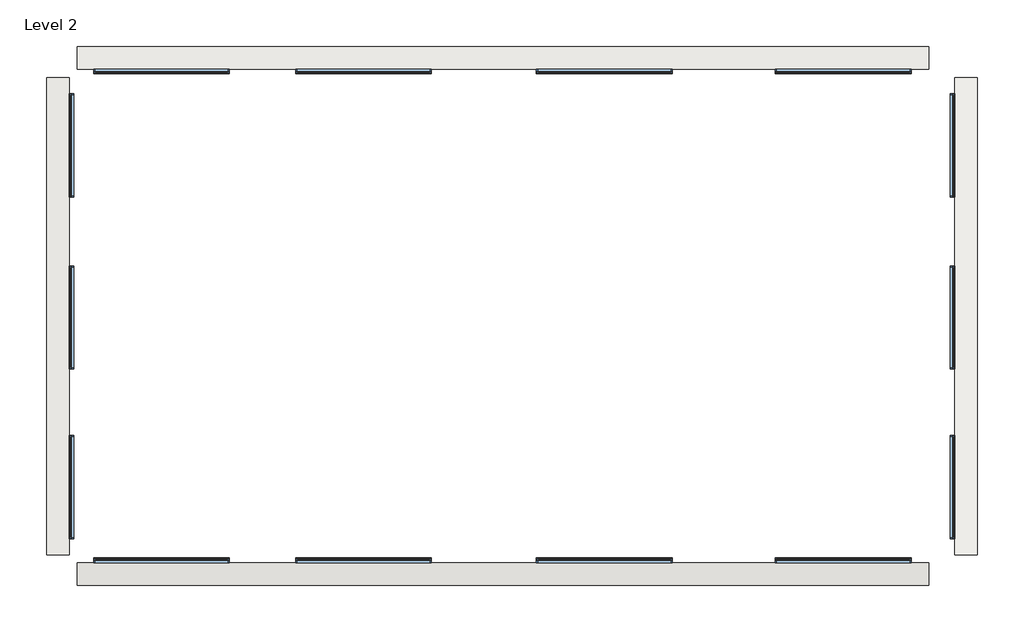
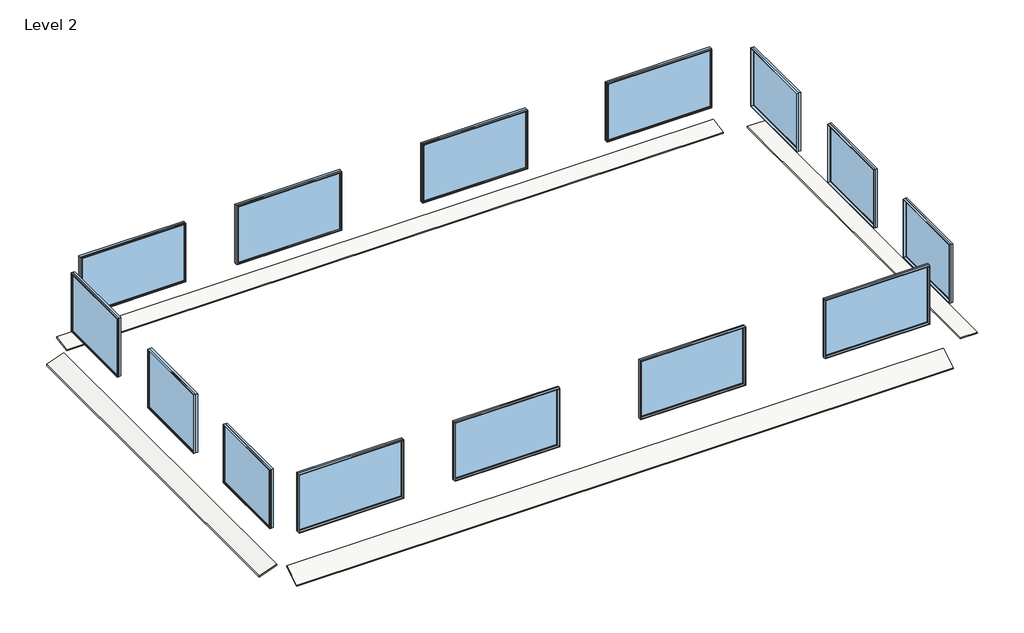
# One storey: 14 windows, 4 roofs.
"""IFC4 building model written with IfcOpenShell, lengths in millimetres."""

import ifcopenshell
import ifcopenshell.guid

model = None  # the IFC model being written
_history = None  # IfcOwnerHistory: only IFC2X3 demands one
_inside = {}  # id of a spatial element -> (the spatial element, [elements in it])
_under = {}  # id of a project, library or spatial element -> (it, [spatial elements below it])
_declared = {}  # id of a project -> (the project, [libraries it declares])
_typed = {}  # id of a type object -> (the type object, [elements of that type])
_made_of = {}  # id of a material, layer set ... -> (it, [elements and type objects made of it])


def new_model(schema):
    """Start an empty IFC model of exactly this schema.

    Asked for "IFC4X3", IfcOpenShell would pick the latest addendum, in which some entities
    have other attributes; the version numbers below select the first issue.
    IFC2X3 requires an IfcOwnerHistory on every rooted entity: one is made here for all.
    """
    global model, _history
    if schema == "IFC4X3":
        model = ifcopenshell.file(schema_version=(4, 3, 0, 0))
    else:
        model = ifcopenshell.file(schema=schema)
    _inside.clear()
    _under.clear()
    _declared.clear()
    _typed.clear()
    _made_of.clear()
    _history = None
    if model.schema == "IFC2X3":
        org = make("IfcOrganization", Name="unknown")
        user = make(
            "IfcPersonAndOrganization",
            ThePerson=make("IfcPerson", FamilyName="unknown"),
            TheOrganization=org,
        )
        app = make(
            "IfcApplication",
            ApplicationDeveloper=org,
            Version="unknown",
            ApplicationFullName="unknown",
            ApplicationIdentifier="unknown",
        )
        _history = make(
            "IfcOwnerHistory",
            OwningUser=user,
            OwningApplication=app,
            ChangeAction="ADDED",
            CreationDate=0,
        )
    return model


def make(cls, **values):
    """One entity of the class cls with the attributes given. An attribute that is None is left unset."""
    return model.create_entity(
        cls, **{name: value for name, value in values.items() if value is not None}
    )


def rooted(cls, **values):
    """An entity with a GlobalId (a new one), such as an element, a storey or a relation."""
    return make(cls, GlobalId=ifcopenshell.guid.new(), OwnerHistory=_history, **values)


def si_unit(unit_type, name, prefix=None):
    """IfcSIUnit, for example si_unit("LENGTHUNIT", "METRE", prefix="MILLI")."""
    return make("IfcSIUnit", UnitType=unit_type, Prefix=prefix, Name=name)


def assignment(units):
    """IfcUnitAssignment: the units of a project."""
    return None if units is None else make("IfcUnitAssignment", Units=units)


def point(xyz):
    """IfcCartesianPoint."""
    return None if xyz is None else make("IfcCartesianPoint", Coordinates=xyz)


def direction(xyz):
    """IfcDirection."""
    return None if xyz is None else make("IfcDirection", DirectionRatios=xyz)


def frame(location, z_axis=None, x_axis=None):
    """IfcAxis2Placement3D, a coordinate frame: its origin and axes. An axis left out is left unset."""
    return make(
        "IfcAxis2Placement3D",
        Location=point(location),
        Axis=direction(z_axis),
        RefDirection=direction(x_axis),
    )


def origin():
    """The frame at (0, 0, 0) with its axes left unset."""
    return frame((0.0, 0.0, 0.0))


def place(relative_to, where):
    """IfcLocalPlacement: puts the frame where relative to a parent placement (None: the world)."""
    return make(
        "IfcLocalPlacement", PlacementRelTo=relative_to, RelativePlacement=where
    )


def context(
    kind, dimensions, precision=None, world=None, true_north=None, identifier=None
):
    """IfcGeometricRepresentationContext, for example the 3D "Model" context."""
    return make(
        "IfcGeometricRepresentationContext",
        ContextIdentifier=identifier,
        ContextType=kind,
        CoordinateSpaceDimension=dimensions,
        Precision=precision,
        WorldCoordinateSystem=world,
        TrueNorth=true_north,
    )


def project(units=None, contexts=None):
    """IfcProject with its units and contexts."""
    return rooted(
        "IfcProject",
        Name="project",
        RepresentationContexts=contexts,
        UnitsInContext=assignment(units),
    )


def spatial(cls, under=None, at=None, **own):
    """A site, building, storey or space (cls), placed at a placement, below another one or the project."""
    s = rooted(cls, ObjectPlacement=at, **own)
    if under is not None:
        _under.setdefault(under.id(), (under, []))[1].append(s)
    return s


def polyline(points):
    """IfcPolyline through the points."""
    return make("IfcPolyline", Points=[point(p) for p in points])


def outline(outer, holes=None, kind="AREA"):
    """IfcArbitraryClosedProfileDef: a profile drawn as a closed curve; with holes, ...WithVoids."""
    if holes is None:
        return make("IfcArbitraryClosedProfileDef", ProfileType=kind, OuterCurve=outer)
    return make(
        "IfcArbitraryProfileDefWithVoids",
        ProfileType=kind,
        OuterCurve=outer,
        InnerCurves=holes,
    )


def extrude(swept, where, along, depth):
    """IfcExtrudedAreaSolid: the profile swept, set in the frame where, extruded along a direction by depth."""
    return make(
        "IfcExtrudedAreaSolid",
        SweptArea=swept,
        Position=where,
        ExtrudedDirection=direction(along),
        Depth=depth,
    )


def shape(context_of_items, identifier, shape_type, items):
    """IfcShapeRepresentation: the items that make up one representation, for example the "Body"."""
    return make(
        "IfcShapeRepresentation",
        ContextOfItems=context_of_items,
        RepresentationIdentifier=identifier,
        RepresentationType=shape_type,
        Items=items,
    )


def source(mapping_origin, context_of_items, identifier, shape_type, items):
    """IfcRepresentationMap: a shape defined once, which mapped items show again and again."""
    return make(
        "IfcRepresentationMap",
        MappingOrigin=mapping_origin,
        MappedRepresentation=shape(context_of_items, identifier, shape_type, items),
    )


def transform(
    local_origin,
    x_axis=None,
    y_axis=None,
    z_axis=None,
    scale=None,
    scale2=None,
    scale3=None,
    uniform=True,
):
    """IfcCartesianTransformationOperator3D, or its non-uniform kind. x_axis, y_axis, z_axis: its Axis1, 2, 3."""
    if uniform:
        return make(
            "IfcCartesianTransformationOperator3D",
            Axis1=direction(x_axis),
            Axis2=direction(y_axis),
            LocalOrigin=point(local_origin),
            Scale=scale,
            Axis3=direction(z_axis),
        )
    return make(
        "IfcCartesianTransformationOperator3DnonUniform",
        Axis1=direction(x_axis),
        Axis2=direction(y_axis),
        LocalOrigin=point(local_origin),
        Scale=scale,
        Axis3=direction(z_axis),
        Scale2=scale2,
        Scale3=scale3,
    )


def mapped(mapping_source, mapping_target):
    """IfcMappedItem: shows the shape of a source again, moved by a transform."""
    return make(
        "IfcMappedItem", MappingSource=mapping_source, MappingTarget=mapping_target
    )


def made_of(thing, what):
    """Note that an element or type object is made of a material, layer set ...; save() writes the relation."""
    if what is not None:
        _made_of.setdefault(what.id(), (what, []))[1].append(thing)
    return thing


def element(
    cls,
    number,
    at=None,
    inside=None,
    cuts=None,
    type_object=None,
    material=None,
    context=None,
    identifier="Body",
    shape_type=None,
    held_by="IfcProductDefinitionShape",
    body=None,
    shapes=None,
    **own,
):
    """One element of the class cls, such as IfcWall. Its Tag is "e" and its number.

    at: its placement. inside: the storey or other place that contains it. cuts: it is an
    opening in that element (IfcRelVoidsElement). A single representation is given by context,
    identifier, shape_type and body (its items); several are given by shapes. held_by: the class
    of the entity that holds the representations. save() writes the other relations.
    """
    e = rooted(cls, Tag="e%d" % number, ObjectPlacement=at, **own)
    if body is not None:
        shapes = [shape(context, identifier, shape_type, body)]
    if shapes is not None:
        e.Representation = make(held_by, Representations=shapes)
    if inside is not None:
        _inside.setdefault(inside.id(), (inside, []))[1].append(e)
    if cuts is not None:
        rooted(
            "IfcRelVoidsElement", RelatingBuildingElement=cuts, RelatedOpeningElement=e
        )
    if type_object is not None:
        _typed.setdefault(type_object.id(), (type_object, []))[1].append(e)
    return made_of(e, material)


def aggregate(whole, parts):
    """IfcRelAggregates: a whole, such as a stair, and the parts it consists of."""
    return rooted("IfcRelAggregates", RelatingObject=whole, RelatedObjects=parts)


def save(model, path):
    """Write the relations noted so far, then the file.

    IfcRelAggregates (storeys below a building ...), IfcRelContainedInSpatialStructure (elements
    in a storey), IfcRelDefinesByType, IfcRelAssociatesMaterial and IfcRelDeclares: one each for
    every whole, place, type object, material and project.
    """
    for whole, parts in _under.values():
        aggregate(whole, parts)
    for where, things in _inside.values():
        rooted(
            "IfcRelContainedInSpatialStructure",
            RelatedElements=things,
            RelatingStructure=where,
        )
    for kind, things in _typed.values():
        rooted("IfcRelDefinesByType", RelatedObjects=things, RelatingType=kind)
    for what, things in _made_of.values():
        rooted("IfcRelAssociatesMaterial", RelatedObjects=things, RelatingMaterial=what)
    for by, libraries in _declared.values():
        rooted("IfcRelDeclares", RelatingContext=by, RelatedDefinitions=libraries)
    model.write(path)


def m_fixed_2500x_4228mm_fd5e51e7(model_context):
    return source(origin(), model_context, "Body", "SweptSolid", [
        extrude(outline(polyline([(-2050.8, 54.2), (2050.8, 54.2), (2050.8, 42.2), (-2050.8, 42.2), (-2050.8, 54.2)])), frame((0.0, 0.0, 368.0), z_axis=(0.0, 0.0, 1.0), x_axis=(1.0, 0.0, 0.0)), (0.0, 0.0, 1.0), 2374.0),
        extrude(outline(polyline([(2786.0, -2094.8), (324.0, -2094.8), (324.0, 2094.8), (2786.0, 2094.8), (2786.0, -2094.8)]), holes=[polyline([(2742.0, -2050.8), (2742.0, 2050.8), (368.0, 2050.8), (368.0, -2050.8), (2742.0, -2050.8)])]), frame((0.0, 26.2, 0.0), z_axis=(0.0, 1.0, 0.0), x_axis=(0.0, 0.0, 1.0)), (0.0, 0.0, 1.0), 44.0),
        extrude(outline(polyline([(2805.0, -2113.8), (305.0, -2113.8), (305.0, 2113.8), (2805.0, 2113.8), (2805.0, -2113.8)]), holes=[polyline([(2786.0, -2094.8), (2786.0, 2094.8), (324.0, 2094.8), (324.0, -2094.8), (2786.0, -2094.8)])]), frame((0.0, 26.2, 0.0), z_axis=(0.0, 1.0, 0.0), x_axis=(0.0, 0.0, 1.0)), (0.0, 0.0, 1.0), 63.0),
        extrude(outline(polyline([(2805.0, -2113.8), (305.0, -2113.8), (305.0, 2113.8), (2805.0, 2113.8), (2805.0, -2113.8)]), holes=[polyline([(2773.0, -2081.8), (2773.0, 2081.8), (337.0, 2081.8), (337.0, -2081.8), (2773.0, -2081.8)])]), frame((0.0, -63.2, 0.0), z_axis=(0.0, 1.0, 0.0), x_axis=(0.0, 0.0, 1.0)), (0.0, 0.0, 1.0), 89.4),
    ])


def m_fixed_2500x_4228mm_f14c179f(model_context):
    return source(origin(), model_context, "Body", "SweptSolid", [
        extrude(outline(polyline([(-2050.8, -54.2), (-2050.8, -42.2), (2050.8, -42.2), (2050.8, -54.2), (-2050.8, -54.2)])), frame((0.0, 0.0, 368.0), z_axis=(0.0, 0.0, 1.0), x_axis=(1.0, 0.0, 0.0)), (0.0, 0.0, 1.0), 2374.0),
        extrude(outline(polyline([(2786.0, -2094.8), (324.0, -2094.8), (324.0, 2094.8), (2786.0, 2094.8), (2786.0, -2094.8)]), holes=[polyline([(2742.0, -2050.8), (2742.0, 2050.8), (368.0, 2050.8), (368.0, -2050.8), (2742.0, -2050.8)])]), frame((0.0, -70.2, 0.0), z_axis=(0.0, 1.0, 0.0), x_axis=(0.0, 0.0, 1.0)), (0.0, 0.0, 1.0), 44.0),
        extrude(outline(polyline([(2805.0, -2113.8), (305.0, -2113.8), (305.0, 2113.8), (2805.0, 2113.8), (2805.0, -2113.8)]), holes=[polyline([(2786.0, -2094.8), (2786.0, 2094.8), (324.0, 2094.8), (324.0, -2094.8), (2786.0, -2094.8)])]), frame((0.0, -89.2, 0.0), z_axis=(0.0, 1.0, 0.0), x_axis=(0.0, 0.0, 1.0)), (0.0, 0.0, 1.0), 63.0),
        extrude(outline(polyline([(2805.0, -2113.8), (305.0, -2113.8), (305.0, 2113.8), (2805.0, 2113.8), (2805.0, -2113.8)]), holes=[polyline([(2773.0, -2081.8), (2773.0, 2081.8), (337.0, 2081.8), (337.0, -2081.8), (2773.0, -2081.8)])]), frame((0.0, -26.2, 0.0), z_axis=(0.0, 1.0, 0.0), x_axis=(0.0, 0.0, 1.0)), (0.0, 0.0, 1.0), 89.4),
    ])


def m_fixed_2500x_3220mm_df94f4d0(model_context):
    return source(origin(), model_context, "Body", "SweptSolid", [
        extrude(outline(polyline([(-1546.8, 54.2), (1546.8, 54.2), (1546.8, 42.2), (-1546.8, 42.2), (-1546.8, 54.2)])), frame((0.0, 0.0, 368.0), z_axis=(0.0, 0.0, 1.0), x_axis=(1.0, 0.0, 0.0)), (0.0, 0.0, 1.0), 2374.0),
        extrude(outline(polyline([(2786.0, -1590.8), (324.0, -1590.8), (324.0, 1590.8), (2786.0, 1590.8), (2786.0, -1590.8)]), holes=[polyline([(2742.0, -1546.8), (2742.0, 1546.8), (368.0, 1546.8), (368.0, -1546.8), (2742.0, -1546.8)])]), frame((0.0, 26.2, 0.0), z_axis=(0.0, 1.0, 0.0), x_axis=(0.0, 0.0, 1.0)), (0.0, 0.0, 1.0), 44.0),
        extrude(outline(polyline([(2805.0, -1609.8), (305.0, -1609.8), (305.0, 1609.8), (2805.0, 1609.8), (2805.0, -1609.8)]), holes=[polyline([(2786.0, -1590.8), (2786.0, 1590.8), (324.0, 1590.8), (324.0, -1590.8), (2786.0, -1590.8)])]), frame((0.0, 26.2, 0.0), z_axis=(0.0, 1.0, 0.0), x_axis=(0.0, 0.0, 1.0)), (0.0, 0.0, 1.0), 63.0),
        extrude(outline(polyline([(2805.0, -1609.8), (305.0, -1609.8), (305.0, 1609.8), (2805.0, 1609.8), (2805.0, -1609.8)]), holes=[polyline([(2773.0, -1577.8), (2773.0, 1577.8), (337.0, 1577.8), (337.0, -1577.8), (2773.0, -1577.8)])]), frame((0.0, -63.2, 0.0), z_axis=(0.0, 1.0, 0.0), x_axis=(0.0, 0.0, 1.0)), (0.0, 0.0, 1.0), 89.4),
    ])


def m_fixed_2500x_3220mm_8b997f8c(model_context):
    return source(origin(), model_context, "Body", "SweptSolid", [
        extrude(outline(polyline([(-1546.8, -54.2), (-1546.8, -42.2), (1546.8, -42.2), (1546.8, -54.2), (-1546.8, -54.2)])), frame((0.0, 0.0, 368.0), z_axis=(0.0, 0.0, 1.0), x_axis=(1.0, 0.0, 0.0)), (0.0, 0.0, 1.0), 2374.0),
        extrude(outline(polyline([(2786.0, -1590.8), (324.0, -1590.8), (324.0, 1590.8), (2786.0, 1590.8), (2786.0, -1590.8)]), holes=[polyline([(2742.0, -1546.8), (2742.0, 1546.8), (368.0, 1546.8), (368.0, -1546.8), (2742.0, -1546.8)])]), frame((0.0, -70.2, 0.0), z_axis=(0.0, 1.0, 0.0), x_axis=(0.0, 0.0, 1.0)), (0.0, 0.0, 1.0), 44.0),
        extrude(outline(polyline([(2805.0, -1609.8), (305.0, -1609.8), (305.0, 1609.8), (2805.0, 1609.8), (2805.0, -1609.8)]), holes=[polyline([(2786.0, -1590.8), (2786.0, 1590.8), (324.0, 1590.8), (324.0, -1590.8), (2786.0, -1590.8)])]), frame((0.0, -89.2, 0.0), z_axis=(0.0, 1.0, 0.0), x_axis=(0.0, 0.0, 1.0)), (0.0, 0.0, 1.0), 63.0),
        extrude(outline(polyline([(2805.0, -1609.8), (305.0, -1609.8), (305.0, 1609.8), (2805.0, 1609.8), (2805.0, -1609.8)]), holes=[polyline([(2773.0, -1577.8), (2773.0, 1577.8), (337.0, 1577.8), (337.0, -1577.8), (2773.0, -1577.8)])]), frame((0.0, -26.2, 0.0), z_axis=(0.0, 1.0, 0.0), x_axis=(0.0, 0.0, 1.0)), (0.0, 0.0, 1.0), 89.4),
    ])


model = new_model("IFC4")

# Units and contexts
model_context = context("Model", 3, world=origin())
ifc_project = project(units=[si_unit("LENGTHUNIT", "METRE", prefix="MILLI")], contexts=[model_context])

# Site, building, storey
site = spatial("IfcSite", under=ifc_project)
building = spatial("IfcBuilding", under=site)
storey = spatial("IfcBuildingStorey", under=building, Name="Level 2", Elevation=3962.4)

# Roofs
placement = place(None, origin())
element("IfcRoof", 1, ObjectType="Shading devices - 50mm", at=placement, inside=storey, context=model_context, shape_type="SweptSolid", body=[
    extrude(outline(polyline([(-4795.4197783, 3248.2548116), (-4095.4197783, 3652.4), (-4095.4197783, 3594.6649731), (-4795.4197783, 3190.5197846), (-4795.4197783, 3248.2548116)])), frame((1746.464681, 0.0, 0.0), z_axis=(1.0, 0.0, 0.0), x_axis=(0.0, 1.0, 0.0)), (0.0, 0.0, 1.0), 26500.0),
])
element("IfcRoof", 2, ObjectType="Shading devices - 50mm", at=placement, inside=storey, context=model_context, shape_type="SweptSolid", body=[
    extrude(outline(polyline([(29068.464681, 11030.5802217), (29768.464681, 11030.5802217), (29768.464681, -3843.0197783), (29068.464681, -3843.0197783), (29068.464681, 11030.5802217)])), frame((0.0, 0.0, 3602.4), z_axis=(0.0, 0.0, 1.0), x_axis=(1.0, 0.0, 0.0)), (0.0, 0.0, 1.0), 50.0),
])
element("IfcRoof", 3, ObjectType="Shading devices - 50mm", at=placement, inside=storey, context=model_context, shape_type="SweptSolid", body=[
    extrude(outline(polyline([(11296.9802217, 3529.7424441), (11996.9802217, 3653.1713306), (11996.9802217, 3602.4), (11296.9802217, 3478.9711135), (11296.9802217, 3529.7424441)])), frame((1746.464681, 0.0, 0.0), z_axis=(1.0, 0.0, 0.0), x_axis=(0.0, 1.0, 0.0)), (0.0, 0.0, 1.0), 26500.0),
])
element("IfcRoof", 4, ObjectType="Shading devices - 50mm", at=placement, inside=storey, context=model_context, shape_type="SweptSolid", body=[
    extrude(outline(polyline([(3652.4, 1484.064681), (3397.620836, 784.064681), (3344.4119474, 784.064681), (3599.1911114, 1484.064681), (3652.4, 1484.064681)])), frame((0.0, -3843.0197783, 0.0), z_axis=(0.0, 1.0, 0.0), x_axis=(0.0, 0.0, 1.0)), (0.0, 0.0, 1.0), 14873.6),
])

# Windows
m_fixed_2500x_4228mm_shape = m_fixed_2500x_4228mm_fd5e51e7(model_context)
element("IfcWindow", 5, ObjectType="M_Fixed : 2500X 4228mm", at=placement, inside=storey, context=model_context, shape_type="MappedRepresentation", body=[
    mapped(m_fixed_2500x_4228mm_shape, transform((4360.264681, 11233.7802217, 4557.4), x_axis=(-1.0, 0.0, 0.0), y_axis=(0.0, -1.0, 0.0), z_axis=(0.0, 0.0, 1.0))),
])
element("IfcWindow", 6, ObjectType="M_Fixed : 2500X 4228mm", at=placement, inside=storey, context=model_context, shape_type="MappedRepresentation", body=[
    mapped(m_fixed_2500x_4228mm_shape, transform((10652.264681, 11233.7802217, 4557.4), x_axis=(-1.0, 0.0, 0.0), y_axis=(0.0, -1.0, 0.0), z_axis=(0.0, 0.0, 1.0))),
])
element("IfcWindow", 7, ObjectType="M_Fixed : 2500X 4228mm", at=placement, inside=storey, context=model_context, shape_type="MappedRepresentation", body=[
    mapped(m_fixed_2500x_4228mm_shape, transform((18152.264681, 11233.7802217, 4557.4), x_axis=(-1.0, 0.0, 0.0), y_axis=(0.0, -1.0, 0.0), z_axis=(0.0, 0.0, 1.0))),
])
element("IfcWindow", 8, ObjectType="M_Fixed : 2500X 4228mm", at=placement, inside=storey, context=model_context, shape_type="MappedRepresentation", body=[
    mapped(m_fixed_2500x_4228mm_shape, transform((25592.264681, 11233.7802217, 4557.4), x_axis=(-1.0, 0.0, 0.0), y_axis=(0.0, -1.0, 0.0), z_axis=(0.0, 0.0, 1.0))),
])
m_fixed_2500x_4228mm_2_shape = m_fixed_2500x_4228mm_f14c179f(model_context)
element("IfcWindow", 9, ObjectType="M_Fixed : 2500X 4228mm", at=placement, inside=storey, context=model_context, shape_type="MappedRepresentation", body=[
    mapped(m_fixed_2500x_4228mm_2_shape, transform((4360.264681, -4032.2197783, 4557.4), x_axis=(-1.0, 0.0, 0.0), y_axis=(0.0, -1.0, 0.0), z_axis=(0.0, 0.0, 1.0))),
])
element("IfcWindow", 10, ObjectType="M_Fixed : 2500X 4228mm", at=placement, inside=storey, context=model_context, shape_type="MappedRepresentation", body=[
    mapped(m_fixed_2500x_4228mm_2_shape, transform((10652.264681, -4032.2197783, 4557.4), x_axis=(-1.0, 0.0, 0.0), y_axis=(0.0, -1.0, 0.0), z_axis=(0.0, 0.0, 1.0))),
])
element("IfcWindow", 11, ObjectType="M_Fixed : 2500X 4228mm", at=placement, inside=storey, context=model_context, shape_type="MappedRepresentation", body=[
    mapped(m_fixed_2500x_4228mm_2_shape, transform((18152.264681, -4032.2197783, 4557.4), x_axis=(-1.0, 0.0, 0.0), y_axis=(0.0, -1.0, 0.0), z_axis=(0.0, 0.0, 1.0))),
])
element("IfcWindow", 12, ObjectType="M_Fixed : 2500X 4228mm", at=placement, inside=storey, context=model_context, shape_type="MappedRepresentation", body=[
    mapped(m_fixed_2500x_4228mm_2_shape, transform((25592.264681, -4032.2197783, 4557.4), x_axis=(-1.0, 0.0, 0.0), y_axis=(0.0, -1.0, 0.0), z_axis=(0.0, 0.0, 1.0))),
])
m_fixed_2500x_3220mm_shape = m_fixed_2500x_3220mm_df94f4d0(model_context)
element("IfcWindow", 13, ObjectType="M_Fixed : 2500x 3220mm", at=placement, inside=storey, context=model_context, shape_type="MappedRepresentation", body=[
    mapped(m_fixed_2500x_3220mm_shape, transform((1573.264681, 8920.7802217, 4559.8), x_axis=(0.0, 1.0, 0.0), y_axis=(-1.0, 0.0, 0.0), z_axis=(0.0, 0.0, 1.0))),
])
element("IfcWindow", 14, ObjectType="M_Fixed : 2500x 3220mm", at=placement, inside=storey, context=model_context, shape_type="MappedRepresentation", body=[
    mapped(m_fixed_2500x_3220mm_shape, transform((1573.264681, 3552.7802217, 4559.8), x_axis=(0.0, 1.0, 0.0), y_axis=(-1.0, 0.0, 0.0), z_axis=(0.0, 0.0, 1.0))),
])
element("IfcWindow", 15, ObjectType="M_Fixed : 2500x 3220mm", at=placement, inside=storey, context=model_context, shape_type="MappedRepresentation", body=[
    mapped(m_fixed_2500x_3220mm_shape, transform((1573.264681, -1733.2197783, 4559.8), x_axis=(0.0, 1.0, 0.0), y_axis=(-1.0, 0.0, 0.0), z_axis=(0.0, 0.0, 1.0))),
])
m_fixed_2500x_3220mm_2_shape = m_fixed_2500x_3220mm_8b997f8c(model_context)
element("IfcWindow", 16, ObjectType="M_Fixed : 2500x 3220mm", at=placement, inside=storey, context=model_context, shape_type="MappedRepresentation", body=[
    mapped(m_fixed_2500x_3220mm_2_shape, transform((28979.264681, 8920.7802217, 4559.8), x_axis=(0.0, 1.0, 0.0), y_axis=(-1.0, 0.0, 0.0), z_axis=(0.0, 0.0, 1.0))),
])
element("IfcWindow", 17, ObjectType="M_Fixed : 2500x 3220mm", at=placement, inside=storey, context=model_context, shape_type="MappedRepresentation", body=[
    mapped(m_fixed_2500x_3220mm_2_shape, transform((28979.264681, 3552.7802217, 4559.8), x_axis=(0.0, 1.0, 0.0), y_axis=(-1.0, 0.0, 0.0), z_axis=(0.0, 0.0, 1.0))),
])
element("IfcWindow", 18, ObjectType="M_Fixed : 2500x 3220mm", at=placement, inside=storey, context=model_context, shape_type="MappedRepresentation", body=[
    mapped(m_fixed_2500x_3220mm_2_shape, transform((28979.264681, -1733.2197783, 4559.8), x_axis=(0.0, 1.0, 0.0), y_axis=(-1.0, 0.0, 0.0), z_axis=(0.0, 0.0, 1.0))),
])

save(model, "model.ifc")

# Revit data of these elements
# Type "Shading devices - 50mm"
#   Layers, outside or top first: 50 mm no material (function 1)
# Type "M_Fixed : 2500X 4228mm"
#   Type Mark = "25"
#   Height = 2500 mm
#   Default Sill Height = 305 mm
#   Width = 4227.6 mm
#   Window Inset = 19 mm
#   Frame Exterior Material = Sash
#   Frame Interior Material = Sash
#   Glass Pane Material = Glass
#   Sash = Sash
#   Wall Closure = (empty or 0)
# Type "M_Fixed : 2500x 3220mm"
#   Type Mark = "26"
#   Height = 2500 mm
#   Default Sill Height = 305 mm
#   Width = 3219.6 mm
#   Window Inset = 19 mm
#   Frame Exterior Material = Sash
#   Frame Interior Material = Sash
#   Glass Pane Material = Glass
#   Sash = Sash
#   Wall Closure = (empty or 0)
# Element 1 (IfcRoof, "Shading devices - 50mm")
#   built-in parameter 1001705 = 11.9829 (stored number, unit not read)
#   built-in parameter 1001701 = -2.53242 (stored number, unit not read)
#   built-in parameter 1001710 = 33615
#   Phase Created = New Construction
#   Materials on its faces: "Default Roof"
# Element 2 (IfcRoof, "Shading devices - 50mm")
#   built-in parameter 1001705 = 11.9829 (stored number, unit not read)
#   built-in parameter 1001701 = -1.1811 (stored number, unit not read)
#   built-in parameter 1001710 = 33615
#   Phase Created = New Construction
#   Materials on its faces: "Default Roof"
# Element 3 (IfcRoof, "Shading devices - 50mm")
#   built-in parameter 1001705 = 11.9855 (stored number, unit not read)
#   built-in parameter 1001701 = -1.1811 (stored number, unit not read)
#   built-in parameter 1001710 = 33615
#   Phase Created = New Construction
#   Materials on its faces: "Default Roof"
# Element 4 (IfcRoof, "Shading devices - 50mm")
#   built-in parameter 1001705 = 11.9829 (stored number, unit not read)
#   built-in parameter 1001701 = -2.02752 (stored number, unit not read)
#   built-in parameter 1001710 = 33615
#   Phase Created = New Construction
#   Materials on its faces: "Default Roof"
# Element 5 (IfcWindow, "M_Fixed : 2500X 4228mm")
#   Mark = "1"
#   Phase Created = New Construction
#   Materials on its faces: "Sash", "Glass"
# Element 6 (IfcWindow, "M_Fixed : 2500X 4228mm")
#   Mark = "2"
#   Phase Created = New Construction
#   Materials on its faces: "Sash", "Glass"
# Element 7 (IfcWindow, "M_Fixed : 2500X 4228mm")
#   Mark = "3"
#   Phase Created = New Construction
#   Materials on its faces: "Sash", "Glass"
# Element 8 (IfcWindow, "M_Fixed : 2500X 4228mm")
#   Mark = "4"
#   Phase Created = New Construction
#   Materials on its faces: "Sash", "Glass"
# Element 9 (IfcWindow, "M_Fixed : 2500X 4228mm")
#   Mark = "5"
#   Phase Created = New Construction
#   Materials on its faces: "Sash", "Glass"
# Element 10 (IfcWindow, "M_Fixed : 2500X 4228mm")
#   Mark = "6"
#   Phase Created = New Construction
#   Materials on its faces: "Sash", "Glass"
# Element 11 (IfcWindow, "M_Fixed : 2500X 4228mm")
#   Mark = "7"
#   Phase Created = New Construction
#   Materials on its faces: "Sash", "Glass"
# Element 12 (IfcWindow, "M_Fixed : 2500X 4228mm")
#   Mark = "8"
#   Phase Created = New Construction
#   Materials on its faces: "Sash", "Glass"
# Element 13 (IfcWindow, "M_Fixed : 2500x 3220mm")
#   Mark = "29"
#   Phase Created = New Construction
#   Materials on its faces: "Sash", "Glass"
# Element 14 (IfcWindow, "M_Fixed : 2500x 3220mm")
#   Mark = "33"
#   Phase Created = New Construction
#   Materials on its faces: "Sash", "Glass"
# Element 15 (IfcWindow, "M_Fixed : 2500x 3220mm")
#   Mark = "34"
#   Phase Created = New Construction
#   Materials on its faces: "Sash", "Glass"
# Element 16 (IfcWindow, "M_Fixed : 2500x 3220mm")
#   Mark = "20"
#   Phase Created = New Construction
#   Materials on its faces: "Sash", "Glass"
# Element 17 (IfcWindow, "M_Fixed : 2500x 3220mm")
#   Mark = "21"
#   Phase Created = New Construction
#   Materials on its faces: "Sash", "Glass"
# Element 18 (IfcWindow, "M_Fixed : 2500x 3220mm")
#   Mark = "22"
#   Phase Created = New Construction
#   Materials on its faces: "Sash", "Glass"
# Materials
#   "Sash": class "Wood", colour RGB 136 99 55, transparency 0
#   "Glass": class "Glass", colour RGB 0 128 192, transparency 0.9, Description = "Soda Lime Glass", Cost = 0
#   "Default Roof": class "Miscellaneous", colour RGB 0 127 0, transparency 0, Cost = 0
# Room at (7702.307, 8283.876) mm, phase "New Construction", upper level "Roof Level", upper offset 0 mm, lower offset 0 mm
#   Number = "9"
#   Name = "Room"
# Room at (8641.307, 981.272) mm, phase "New Construction", upper level "Roof Level", upper offset 0 mm, lower offset 0 mm
#   Number = "10"
#   Name = "Room"
